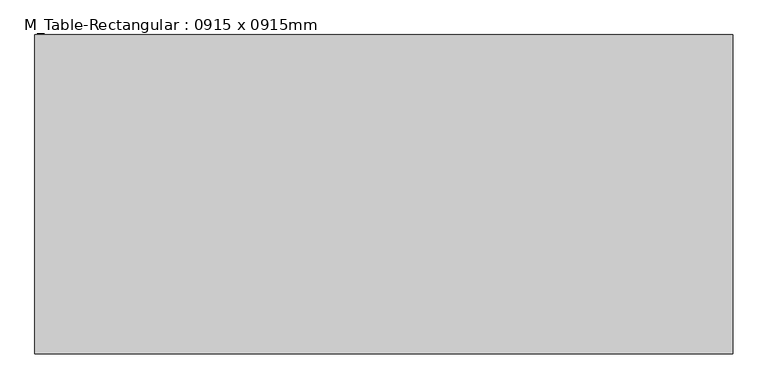
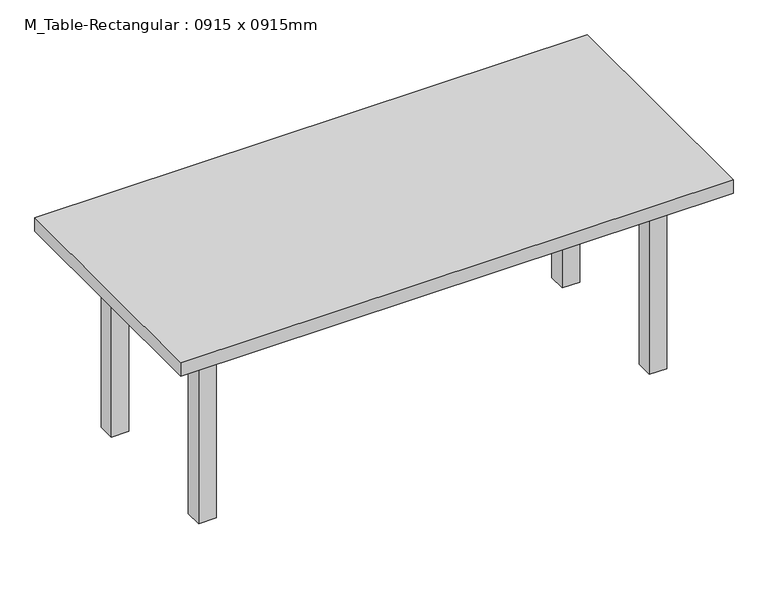
"""IFC4 building model written with IfcOpenShell, lengths in millimetres: furniture geometry, M_Table-Rectangular : 0915 x 0915mm."""

from ifc_helpers import new_model, si_unit, frame, origin, origin_with_axes, place, context, project, spatial, polyline, outline, extrude, source, transform, mapped, element, save


def m_table_rectangular_0915_x_0915mm_cd8de91e(model_context):
    return source(origin(), model_context, "Body", "SweptSolid", [
        extrude(outline(polyline([(784.1, 267.0), (784.1, 241.6), (-784.1, 241.6), (-784.1, 267.0), (784.1, 267.0)])), frame((0.0, 0.0, 609.6), z_axis=(0.0, 0.0, 1.0), x_axis=(1.0, 0.0, 0.0)), (0.0, 0.0, 1.0), 101.6),
        extrude(outline(polyline([(784.1, -267.0), (-784.1, -267.0), (-784.1, -241.6), (784.1, -241.6), (784.1, -267.0)])), frame((0.0, 0.0, 609.6), z_axis=(0.0, 0.0, 1.0), x_axis=(1.0, 0.0, 0.0)), (0.0, 0.0, 1.0), 101.6),
        extrude(outline(polyline([(-796.8, -241.6), (-822.2, -241.6), (-822.2, 241.6), (-796.8, 241.6), (-796.8, -241.6)])), frame((0.0, 0.0, 609.6), z_axis=(0.0, 0.0, 1.0), x_axis=(1.0, 0.0, 0.0)), (0.0, 0.0, 1.0), 101.6),
        extrude(outline(polyline([(796.8, -241.6), (796.8, 241.6), (822.2, 241.6), (822.2, -241.6), (796.8, -241.6)])), frame((0.0, 0.0, 609.6), z_axis=(0.0, 0.0, 1.0), x_axis=(1.0, 0.0, 0.0)), (0.0, 0.0, 1.0), 101.6),
        extrude(outline(polyline([(1000.0, 457.5), (1000.0, -457.5), (-1000.0, -457.5), (-1000.0, 457.5), (1000.0, 457.5)])), frame((0.0, 0.0, 711.2), z_axis=(0.0, 0.0, 1.0), x_axis=(1.0, 0.0, 0.0)), (0.0, 0.0, 1.0), 50.8),
        extrude(outline(polyline([(-784.1, 305.1), (-784.1, 241.6), (-847.6, 241.6), (-847.6, 305.1), (-784.1, 305.1)])), origin_with_axes(), (0.0, 0.0, 1.0), 711.2),
        extrude(outline(polyline([(784.1, 305.1), (847.6, 305.1), (847.6, 241.6), (784.1, 241.6), (784.1, 305.1)])), origin_with_axes(), (0.0, 0.0, 1.0), 711.2),
        extrude(outline(polyline([(-784.1, -305.1), (-847.6, -305.1), (-847.6, -241.6), (-784.1, -241.6), (-784.1, -305.1)])), origin_with_axes(), (0.0, 0.0, 1.0), 711.2),
        extrude(outline(polyline([(784.1, -305.1), (784.1, -241.6), (847.6, -241.6), (847.6, -305.1), (784.1, -305.1)])), origin_with_axes(), (0.0, 0.0, 1.0), 711.2),
    ])


if __name__ == "__main__":
    model = new_model("IFC4")
    model_context = context("Model", 3, world=origin())
    ifc_project = project(units=[si_unit("LENGTHUNIT", "METRE", prefix="MILLI")], contexts=[model_context])
    site = spatial("IfcSite", under=ifc_project)
    building = spatial("IfcBuilding", under=site)
    placement = place(None, origin())
    m_table_rectangular_0915_x_0915mm_shape = m_table_rectangular_0915_x_0915mm_cd8de91e(model_context)
    element("IfcFurniture", 1, ObjectType="M_Table-Rectangular : 0915 x 0915mm", at=placement, inside=building, context=model_context, shape_type="MappedRepresentation", body=[
        mapped(m_table_rectangular_0915_x_0915mm_shape, transform((0.0, 0.0, 0.0), x_axis=(1.0, 0.0, 0.0), y_axis=(0.0, 1.0, 0.0), z_axis=(0.0, 0.0, 1.0))),
    ])
    save(model, "model.ifc")

# Revit data of these elements
# Type "M_Table-Rectangular : 0915 x 0915mm"
#   Height = 0.762 m
#   Length = 2 m
#   Width = 0.915 m
#   Base Material = Birch
#   Top Material = Birch
# Element 1 (IfcFurniture, "M_Table-Rectangular : 0915 x 0915mm")
#   Materials on its faces: "Birch"
# Materials
#   "Birch": class "Wood", colour RGB 224 178 126, transparency 0, Description = "Betula Alleghaniensis", Cost = 0
